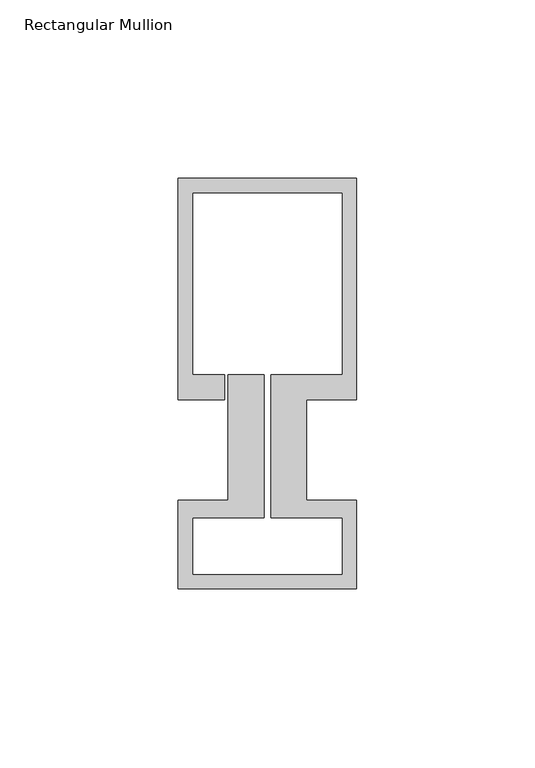
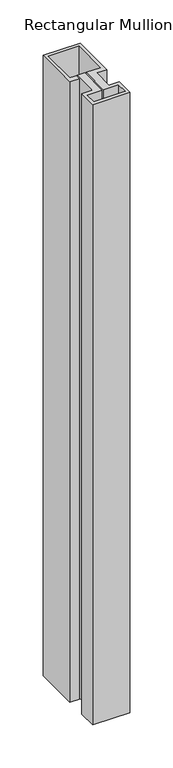
"""IFC4 building model written with IfcOpenShell, lengths in millimetres: member geometry, Rectangular Mullion : Schueco_FWS-50-HI_Tran_CovCap-20mm_Tran-55mm."""

from ifc_helpers import new_model, si_unit, frame, origin, place, context, project, spatial, polyline, outline, extrude, source, transform, mapped, element, save


def rectangular_mullion_31affb63(model_context):
    return source(origin(), model_context, "Body", "SweptSolid", [
        extrude(outline(polyline([(0.0, 90.0), (0.0, 28.0), (-14.0, 28.0), (-14.0, -0.1), (0.0, -0.1), (0.0, -25.0), (-50.0, -25.0), (-50.0, -0.1), (-36.0, -0.1), (-36.0, 35.0), (-26.0, 35.0), (-26.0, -5.0), (-46.0, -5.0), (-46.0, -21.0), (-4.0, -21.0), (-4.0, -5.0), (-24.0, -5.0), (-24.0, 35.0), (-4.0, 35.0), (-4.0, 86.0), (-46.0, 86.0), (-46.0, 35.0), (-37.0, 35.0), (-37.0, 28.0), (-50.0, 28.0), (-50.0, 90.0), (0.0, 90.0)])), frame((0.0, 0.0, -880.0), z_axis=(0.0, 0.0, 1.0), x_axis=(1.0, 0.0, 0.0)), (0.0, 0.0, 1.0), 880.0),
    ])


if __name__ == "__main__":
    model = new_model("IFC4")
    model_context = context("Model", 3, world=origin())
    ifc_project = project(units=[si_unit("LENGTHUNIT", "METRE", prefix="MILLI")], contexts=[model_context])
    site = spatial("IfcSite", under=ifc_project)
    building = spatial("IfcBuilding", under=site)
    placement = place(None, origin())
    rectangular_mullion_shape = rectangular_mullion_31affb63(model_context)
    element("IfcMember", 1, ObjectType="Rectangular Mullion : Schueco_FWS-50-HI_Tran_CovCap-20mm_Tran-55mm", at=placement, inside=building, context=model_context, shape_type="MappedRepresentation", body=[
        mapped(rectangular_mullion_shape, transform((0.0, 0.0, 0.0), x_axis=(1.0, 0.0, 0.0), y_axis=(0.0, 1.0, 0.0), z_axis=(0.0, 0.0, 1.0))),
    ])
    save(model, "model.ifc")

# Revit data of these elements
# Type "Rectangular Mullion : Schueco_FWS-50-HI_Tran_CovCap-20mm_Tran-55mm"
#   Model = "FWS 50.HI"
#   Manufacturer = "Schueco International KG"
#   Type Comments = "Transom"
#   Schueco thermal insulation standard = "Highly thermally insulated"
#   Burglar resistance = "RC 3"
#   Thermal insulation = "to 0.90 W/(m²K)"
#   built-in parameter 1007322 = 0.377297 (stored number, unit not read)
#   built-in parameter 1007321 = 0.0360892 (stored number, unit not read)
#   built-in parameter 1007320 = 0.0360892 (stored number, unit not read)
# Element 1 (IfcMember, "Rectangular Mullion : Schueco_FWS-50-HI_Tran_CovCap-20mm_Tran-55mm")
#   Materials on its faces: "Alu"
# Materials
#   "Alu": class "Glas", colour RGB 140 140 140, transparency 0
